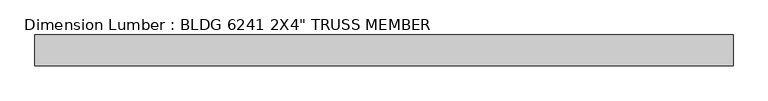
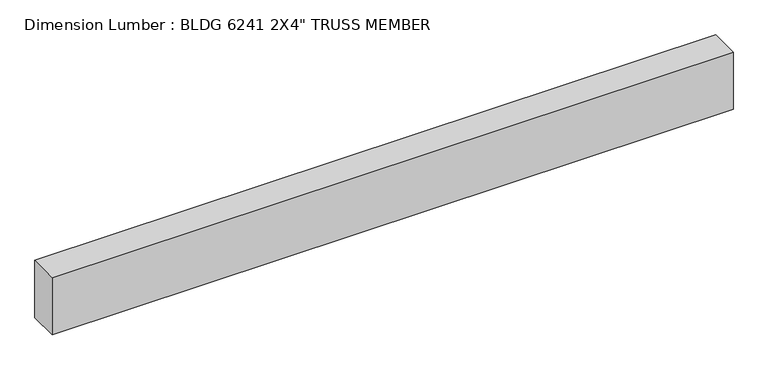
"""IFC4 building model written with IfcOpenShell, lengths in millimetres: beam geometry."""

from ifc_helpers import new_model, si_unit, frame, origin, place, context, project, spatial, polyline, outline, extrude, source, transform, mapped, element, save


def beam_5e172d94(model_context):
    return source(origin(), model_context, "Body", "SweptSolid", [
        extrude(outline(polyline([(595.8662636, 25.4), (595.8662636, -25.4), (-548.2789755, -25.4), (-548.2789755, 25.4), (595.8662636, 25.4)])), frame((0.0, 0.0, -50.8), z_axis=(0.0, 0.0, 1.0), x_axis=(1.0, 0.0, 0.0)), (0.0, 0.0, 1.0), 101.6),
    ])


if __name__ == "__main__":
    model = new_model("IFC4")
    model_context = context("Model", 3, world=origin())
    ifc_project = project(units=[si_unit("LENGTHUNIT", "METRE", prefix="MILLI")], contexts=[model_context])
    site = spatial("IfcSite", under=ifc_project)
    building = spatial("IfcBuilding", under=site)
    placement = place(None, origin())
    beam_shape = beam_5e172d94(model_context)
    element("IfcBeam", 1, ObjectType="Dimension Lumber : BLDG 6241 2X4\" TRUSS MEMBER", at=placement, inside=building, context=model_context, shape_type="MappedRepresentation", body=[
        mapped(beam_shape, transform((0.0, 0.0, 0.0), x_axis=(1.0, 0.0, 0.0), y_axis=(0.0, 1.0, 0.0), z_axis=(0.0, 0.0, 1.0))),
    ])
    save(model, "model.ifc")

# Revit data of these elements
# Type "Dimension Lumber : BLDG 6241 2X4\" TRUSS MEMBER"
#   Assembly Code = "B10"
#   A = 0.273472 SF
#   Length [instance default] = 5' - 0"
#   b = 0' - 2"
#   d = 0' - 4"
#   Structural Material [instance default] = Softwood, Lumber
# Element 1 (IfcBeam, "Dimension Lumber : BLDG 6241 2X4\" TRUSS MEMBER")
#   Materials on its faces: "Softwood, Lumber"
# Materials
#   "Softwood, Lumber": class "Wood", colour RGB 223 192 134, transparency 0, Description = "Pinus Echinata", Cost = 0
